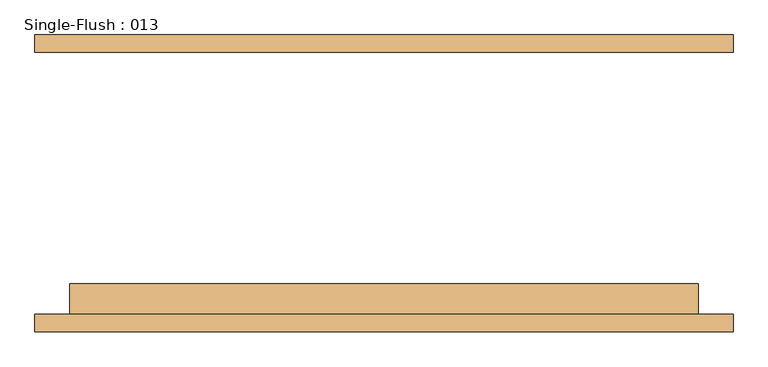
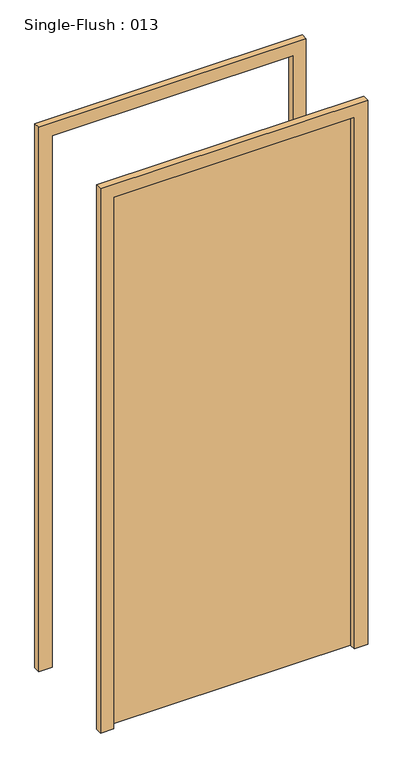
"""IFC4 building model written with IfcOpenShell, lengths in millimetres: door geometry, Single-Flush : 013."""

import ifcopenshell
import ifcopenshell.guid

model = None  # the IFC model being written
_history = None  # IfcOwnerHistory: only IFC2X3 demands one
_inside = {}  # id of a spatial element -> (the spatial element, [elements in it])
_under = {}  # id of a project, library or spatial element -> (it, [spatial elements below it])
_declared = {}  # id of a project -> (the project, [libraries it declares])
_typed = {}  # id of a type object -> (the type object, [elements of that type])
_made_of = {}  # id of a material, layer set ... -> (it, [elements and type objects made of it])


def new_model(schema):
    """Start an empty IFC model of exactly this schema.

    Asked for "IFC4X3", IfcOpenShell would pick the latest addendum, in which some entities
    have other attributes; the version numbers below select the first issue.
    IFC2X3 requires an IfcOwnerHistory on every rooted entity: one is made here for all.
    """
    global model, _history
    if schema == "IFC4X3":
        model = ifcopenshell.file(schema_version=(4, 3, 0, 0))
    else:
        model = ifcopenshell.file(schema=schema)
    _inside.clear()
    _under.clear()
    _declared.clear()
    _typed.clear()
    _made_of.clear()
    _history = None
    if model.schema == "IFC2X3":
        org = make("IfcOrganization", Name="unknown")
        user = make(
            "IfcPersonAndOrganization",
            ThePerson=make("IfcPerson", FamilyName="unknown"),
            TheOrganization=org,
        )
        app = make(
            "IfcApplication",
            ApplicationDeveloper=org,
            Version="unknown",
            ApplicationFullName="unknown",
            ApplicationIdentifier="unknown",
        )
        _history = make(
            "IfcOwnerHistory",
            OwningUser=user,
            OwningApplication=app,
            ChangeAction="ADDED",
            CreationDate=0,
        )
    return model


def make(cls, **values):
    """One entity of the class cls with the attributes given. An attribute that is None is left unset."""
    return model.create_entity(
        cls, **{name: value for name, value in values.items() if value is not None}
    )


def rooted(cls, **values):
    """An entity with a GlobalId (a new one), such as an element, a storey or a relation."""
    return make(cls, GlobalId=ifcopenshell.guid.new(), OwnerHistory=_history, **values)


def si_unit(unit_type, name, prefix=None):
    """IfcSIUnit, for example si_unit("LENGTHUNIT", "METRE", prefix="MILLI")."""
    return make("IfcSIUnit", UnitType=unit_type, Prefix=prefix, Name=name)


def assignment(units):
    """IfcUnitAssignment: the units of a project."""
    return None if units is None else make("IfcUnitAssignment", Units=units)


def point(xyz):
    """IfcCartesianPoint."""
    return None if xyz is None else make("IfcCartesianPoint", Coordinates=xyz)


def direction(xyz):
    """IfcDirection."""
    return None if xyz is None else make("IfcDirection", DirectionRatios=xyz)


def frame(location, z_axis=None, x_axis=None):
    """IfcAxis2Placement3D, a coordinate frame: its origin and axes. An axis left out is left unset."""
    return make(
        "IfcAxis2Placement3D",
        Location=point(location),
        Axis=direction(z_axis),
        RefDirection=direction(x_axis),
    )


def origin():
    """The frame at (0, 0, 0) with its axes left unset."""
    return frame((0.0, 0.0, 0.0))


def origin_with_axes():
    """The frame at (0, 0, 0) with the z axis (0, 0, 1) and the x axis (1, 0, 0) written out."""
    return frame((0.0, 0.0, 0.0), z_axis=(0.0, 0.0, 1.0), x_axis=(1.0, 0.0, 0.0))


def place(relative_to, where):
    """IfcLocalPlacement: puts the frame where relative to a parent placement (None: the world)."""
    return make(
        "IfcLocalPlacement", PlacementRelTo=relative_to, RelativePlacement=where
    )


def context(
    kind, dimensions, precision=None, world=None, true_north=None, identifier=None
):
    """IfcGeometricRepresentationContext, for example the 3D "Model" context."""
    return make(
        "IfcGeometricRepresentationContext",
        ContextIdentifier=identifier,
        ContextType=kind,
        CoordinateSpaceDimension=dimensions,
        Precision=precision,
        WorldCoordinateSystem=world,
        TrueNorth=true_north,
    )


def project(units=None, contexts=None):
    """IfcProject with its units and contexts."""
    return rooted(
        "IfcProject",
        Name="project",
        RepresentationContexts=contexts,
        UnitsInContext=assignment(units),
    )


def spatial(cls, under=None, at=None, **own):
    """A site, building, storey or space (cls), placed at a placement, below another one or the project."""
    s = rooted(cls, ObjectPlacement=at, **own)
    if under is not None:
        _under.setdefault(under.id(), (under, []))[1].append(s)
    return s


def polyline(points):
    """IfcPolyline through the points."""
    return make("IfcPolyline", Points=[point(p) for p in points])


def outline(outer, holes=None, kind="AREA"):
    """IfcArbitraryClosedProfileDef: a profile drawn as a closed curve; with holes, ...WithVoids."""
    if holes is None:
        return make("IfcArbitraryClosedProfileDef", ProfileType=kind, OuterCurve=outer)
    return make(
        "IfcArbitraryProfileDefWithVoids",
        ProfileType=kind,
        OuterCurve=outer,
        InnerCurves=holes,
    )


def extrude(swept, where, along, depth):
    """IfcExtrudedAreaSolid: the profile swept, set in the frame where, extruded along a direction by depth."""
    return make(
        "IfcExtrudedAreaSolid",
        SweptArea=swept,
        Position=where,
        ExtrudedDirection=direction(along),
        Depth=depth,
    )


def shape(context_of_items, identifier, shape_type, items):
    """IfcShapeRepresentation: the items that make up one representation, for example the "Body"."""
    return make(
        "IfcShapeRepresentation",
        ContextOfItems=context_of_items,
        RepresentationIdentifier=identifier,
        RepresentationType=shape_type,
        Items=items,
    )


def source(mapping_origin, context_of_items, identifier, shape_type, items):
    """IfcRepresentationMap: a shape defined once, which mapped items show again and again."""
    return make(
        "IfcRepresentationMap",
        MappingOrigin=mapping_origin,
        MappedRepresentation=shape(context_of_items, identifier, shape_type, items),
    )


def transform(
    local_origin,
    x_axis=None,
    y_axis=None,
    z_axis=None,
    scale=None,
    scale2=None,
    scale3=None,
    uniform=True,
):
    """IfcCartesianTransformationOperator3D, or its non-uniform kind. x_axis, y_axis, z_axis: its Axis1, 2, 3."""
    if uniform:
        return make(
            "IfcCartesianTransformationOperator3D",
            Axis1=direction(x_axis),
            Axis2=direction(y_axis),
            LocalOrigin=point(local_origin),
            Scale=scale,
            Axis3=direction(z_axis),
        )
    return make(
        "IfcCartesianTransformationOperator3DnonUniform",
        Axis1=direction(x_axis),
        Axis2=direction(y_axis),
        LocalOrigin=point(local_origin),
        Scale=scale,
        Axis3=direction(z_axis),
        Scale2=scale2,
        Scale3=scale3,
    )


def mapped(mapping_source, mapping_target):
    """IfcMappedItem: shows the shape of a source again, moved by a transform."""
    return make(
        "IfcMappedItem", MappingSource=mapping_source, MappingTarget=mapping_target
    )


def made_of(thing, what):
    """Note that an element or type object is made of a material, layer set ...; save() writes the relation."""
    if what is not None:
        _made_of.setdefault(what.id(), (what, []))[1].append(thing)
    return thing


def element(
    cls,
    number,
    at=None,
    inside=None,
    cuts=None,
    type_object=None,
    material=None,
    context=None,
    identifier="Body",
    shape_type=None,
    held_by="IfcProductDefinitionShape",
    body=None,
    shapes=None,
    **own,
):
    """One element of the class cls, such as IfcWall. Its Tag is "e" and its number.

    at: its placement. inside: the storey or other place that contains it. cuts: it is an
    opening in that element (IfcRelVoidsElement). A single representation is given by context,
    identifier, shape_type and body (its items); several are given by shapes. held_by: the class
    of the entity that holds the representations. save() writes the other relations.
    """
    e = rooted(cls, Tag="e%d" % number, ObjectPlacement=at, **own)
    if body is not None:
        shapes = [shape(context, identifier, shape_type, body)]
    if shapes is not None:
        e.Representation = make(held_by, Representations=shapes)
    if inside is not None:
        _inside.setdefault(inside.id(), (inside, []))[1].append(e)
    if cuts is not None:
        rooted(
            "IfcRelVoidsElement", RelatingBuildingElement=cuts, RelatedOpeningElement=e
        )
    if type_object is not None:
        _typed.setdefault(type_object.id(), (type_object, []))[1].append(e)
    return made_of(e, material)


def aggregate(whole, parts):
    """IfcRelAggregates: a whole, such as a stair, and the parts it consists of."""
    return rooted("IfcRelAggregates", RelatingObject=whole, RelatedObjects=parts)


def save(model, path):
    """Write the relations noted so far, then the file.

    IfcRelAggregates (storeys below a building ...), IfcRelContainedInSpatialStructure (elements
    in a storey), IfcRelDefinesByType, IfcRelAssociatesMaterial and IfcRelDeclares: one each for
    every whole, place, type object, material and project.
    """
    for whole, parts in _under.values():
        aggregate(whole, parts)
    for where, things in _inside.values():
        rooted(
            "IfcRelContainedInSpatialStructure",
            RelatedElements=things,
            RelatingStructure=where,
        )
    for kind, things in _typed.values():
        rooted("IfcRelDefinesByType", RelatedObjects=things, RelatingType=kind)
    for what, things in _made_of.values():
        rooted("IfcRelAssociatesMaterial", RelatedObjects=things, RelatingMaterial=what)
    for by, libraries in _declared.values():
        rooted("IfcRelDeclares", RelatingContext=by, RelatedDefinitions=libraries)
    model.write(path)


def single_flush_013_d0afb6d8(model_context):
    return source(origin(), model_context, "Body", "SweptSolid", [
        extrude(outline(polyline([(2184.4, -508.0), (0.0, -508.0), (0.0, -457.2), (2133.6, -457.2), (2133.6, 457.2), (0.0, 457.2), (0.0, 508.0), (2184.4, 508.0), (2184.4, -508.0)])), frame((0.0, -215.9, 0.0), z_axis=(0.0, 1.0, 0.0), x_axis=(0.0, 0.0, 1.0)), (0.0, 0.0, 1.0), 25.4),
        extrude(outline(polyline([(2184.4, 508.0), (2184.4, -508.0), (0.0, -508.0), (0.0, -457.2), (2133.6, -457.2), (2133.6, 457.2), (0.0, 457.2), (0.0, 508.0), (2184.4, 508.0)])), frame((0.0, 190.5, 0.0), z_axis=(0.0, 1.0, 0.0), x_axis=(0.0, 0.0, 1.0)), (0.0, 0.0, 1.0), 25.4),
        extrude(outline(polyline([(457.2, -146.05), (457.2, -190.5), (-457.2, -190.5), (-457.2, -146.05), (457.2, -146.05)])), origin_with_axes(), (0.0, 0.0, 1.0), 2133.6),
    ])


if __name__ == "__main__":
    model = new_model("IFC4")
    model_context = context("Model", 3, world=origin())
    ifc_project = project(units=[si_unit("LENGTHUNIT", "METRE", prefix="MILLI")], contexts=[model_context])
    site = spatial("IfcSite", under=ifc_project)
    building = spatial("IfcBuilding", under=site)
    placement = place(None, origin())
    single_flush_013_shape = single_flush_013_d0afb6d8(model_context)
    element("IfcDoor", 1, ObjectType="Single-Flush : 013", at=placement, inside=building, context=model_context, shape_type="MappedRepresentation", body=[
        mapped(single_flush_013_shape, transform((0.0, 0.0, 0.0), x_axis=(1.0, 0.0, 0.0), y_axis=(0.0, 1.0, 0.0), z_axis=(0.0, 0.0, 1.0))),
    ])
    save(model, "model.ifc")

# Revit data of these elements
# Type "Single-Flush : 013"
#   Type Mark = "013"
#   Construction Type Id = "MDOOR"
#   Assembly Code = "C1020"
#   Analytic Construction = "Metal"
#   Thickness = 0' - 1 3/4"
#   Heat Transfer Coefficient (U) = 3.7021 W/(m²·K)
#   Height = 7' - 0"
#   Trim Projection Ext = 0' - 1"
#   Trim Projection Int = 0' - 1"
#   Trim Width = 0' - 2"
#   Width = 3' - 0"
#   Door Material = 05 - Metal - Steel
#   Frame Material = 05 - Metal - Aluminum
#   Visual Light Transmittance = 0
#   Solar Heat Gain Coefficient = 0
#   Function = (empty or 0)
#   Wall Closure = (empty or 0)
# Element 1 (IfcDoor, "Single-Flush : 013")
#   Materials on its faces: "05 - Metal - Aluminum", "05 - Metal - Steel"
# Materials
#   "05 - Metal - Steel": class "Unassigned", colour RGB 199 199 199, transparency 0, Description = "Steel"
#   "05 - Metal - Aluminum": class "Unassigned", colour RGB 247 247 247, transparency 0, Description = "Aluminum"
